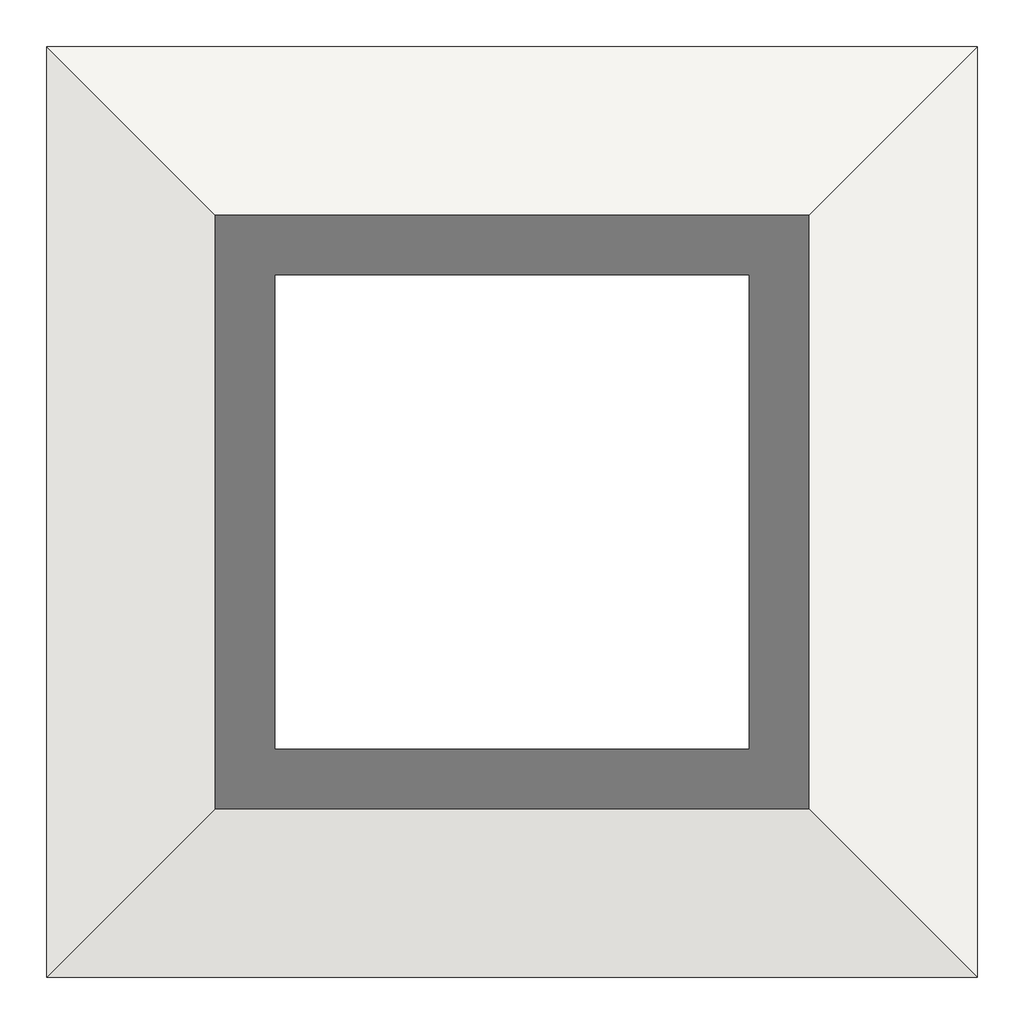
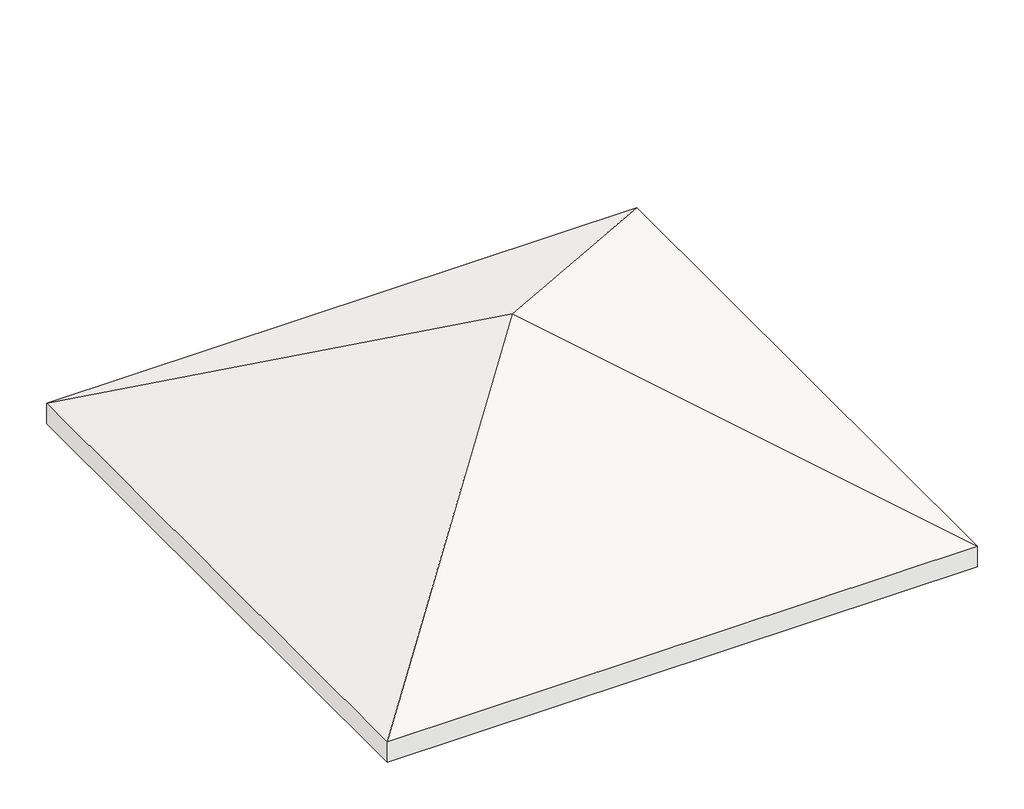
# One storey: 4 beams, 1 roof.
"""IFC4 building model written with IfcOpenShell, lengths in millimetres."""

from ifc_helpers import new_model, si_unit, frame, origin, place, context, project, spatial, polyline, outline, extrude, faceted_brep, element, save

model = new_model("IFC4")

# Units and contexts
model_context = context("Model", 3, world=origin())
ifc_project = project(units=[si_unit("LENGTHUNIT", "METRE", prefix="MILLI")], contexts=[model_context])

# Site, building, storey
site = spatial("IfcSite", under=ifc_project)
building = spatial("IfcBuilding", under=site)
storey = spatial("IfcBuildingStorey", under=building, Name="Nível 2", Elevation=4000.0)

# Beams
placement = place(None, origin())
element("IfcBeam", 1, ObjectType="Concreto-Viga retangular : 400 x 800mm", at=placement, inside=storey, context=model_context, shape_type="SweptSolid", body=[
    extrude(outline(polyline([(-2623.6821965, 6011.329614), (-2623.6821965, 6411.329614), (6776.3178035, 6411.329614), (6776.3178035, 6011.329614), (-2623.6821965, 6011.329614)])), frame((0.0, 0.0, 3200.0), z_axis=(0.0, 0.0, 1.0), x_axis=(1.0, 0.0, 0.0)), (0.0, 0.0, 1.0), 800.0),
])
element("IfcBeam", 2, ObjectType="Concreto-Viga retangular : 400 x 800mm", at=placement, inside=storey, context=model_context, shape_type="SweptSolid", body=[
    extrude(outline(polyline([(7276.3178035, -3488.670386), (6876.3178035, -3488.670386), (6876.3178035, 5911.329614), (7276.3178035, 5911.329614), (7276.3178035, -3488.670386)])), frame((0.0, 0.0, 3200.0), z_axis=(0.0, 0.0, 1.0), x_axis=(1.0, 0.0, 0.0)), (0.0, 0.0, 1.0), 800.0),
])
element("IfcBeam", 3, ObjectType="Concreto-Viga retangular : 400 x 800mm", at=placement, inside=storey, context=model_context, shape_type="SweptSolid", body=[
    extrude(outline(polyline([(-2623.6821965, -3988.670386), (-2623.6821965, -3588.670386), (6776.3178035, -3588.670386), (6776.3178035, -3988.670386), (-2623.6821965, -3988.670386)])), frame((0.0, 0.0, 3200.0), z_axis=(0.0, 0.0, 1.0), x_axis=(1.0, 0.0, 0.0)), (0.0, 0.0, 1.0), 800.0),
])
element("IfcBeam", 4, ObjectType="Concreto-Viga retangular : 400 x 800mm", at=placement, inside=storey, context=model_context, shape_type="SweptSolid", body=[
    extrude(outline(polyline([(-3123.6821965, 5911.329614), (-2723.6821965, 5911.329614), (-2723.6821965, -3488.670386), (-3123.6821965, -3488.670386), (-3123.6821965, 5911.329614)])), frame((0.0, 0.0, 3200.0), z_axis=(0.0, 0.0, 1.0), x_axis=(1.0, 0.0, 0.0)), (0.0, 0.0, 1.0), 800.0),
])

# Roof
element("IfcRoof", 5, ObjectType="Genérico - 400 mm", at=placement, inside=storey, context=model_context, shape_type="Brep", body=[
    faceted_brep([(8276.3178035, 7411.329614, 3440.0), (2076.3178035, 1211.329614, 7019.571669), (-4123.6821965, 7411.329614, 3440.0), (-4123.6821965, -4988.670386, 3440.0), (8276.3178035, -4988.670386, 3440.0), (8276.3178035, 7411.329614, 3901.8802154), (-4123.6821965, 7411.329614, 3901.8802154), (2076.3178035, 1211.329614, 7481.4518843), (-4123.6821965, -4988.670386, 3901.8802154), (8276.3178035, -4988.670386, 3901.8802154)], [[[0, 1, 2]], [[2, 1, 3]], [[3, 1, 4]], [[1, 0, 4]], [[5, 6, 7]], [[6, 8, 7]], [[8, 9, 7]], [[5, 7, 9]], [[2, 6, 5, 0]], [[3, 8, 6, 2]], [[4, 9, 8, 3]], [[0, 5, 9, 4]]]),
])

save(model, "model.ifc")

# Revit data of these elements
# Type "Concreto-Viga retangular : 400 x 800mm"
#   Length [instance default] = 1.524 m
#   b = 0.40 m
#   h = 0.80 m
#   Structural Material [instance default] = Concreto, Moldado in loco, cinza
#   Assembly Code = ""
# Type "Genérico - 400 mm"
#   Layers, outside or top first: 0.40 m no material (function 1)
# Elements 1, 2, 3, 4 (IfcBeam, "Concreto-Viga retangular : 400 x 800mm")
#   Structural Material = Concreto, Moldado in loco, cinza
#   Phase Created = Construção nova
#   Materials on its faces: "Concreto, Moldado in loco, cinza"
# Element 5 (IfcRoof, "Genérico - 400 mm")
#   built-in parameter 1001705 = 24.5454 (stored number, unit not read)
#   built-in parameter 1001701 = -1.83727 (stored number, unit not read)
#   built-in parameter 1001710 = 33615
#   Phase Created = Construção nova
#   Materials on its faces: "Telhado padrão"
# Materials
#   "Concreto, Moldado in loco, cinza": class "Concreto", colour RGB 192 192 192, transparency 0, Description = "Concreto moldado in loco", Cost = 0
#   "Telhado padrão": class "Diversos", colour RGB 0 127 0, transparency 0, Cost = 0
